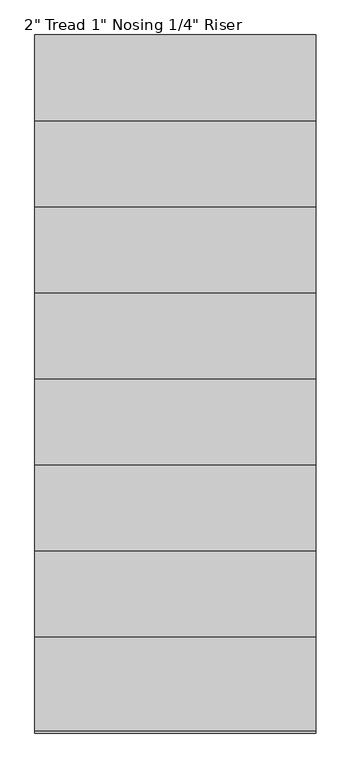
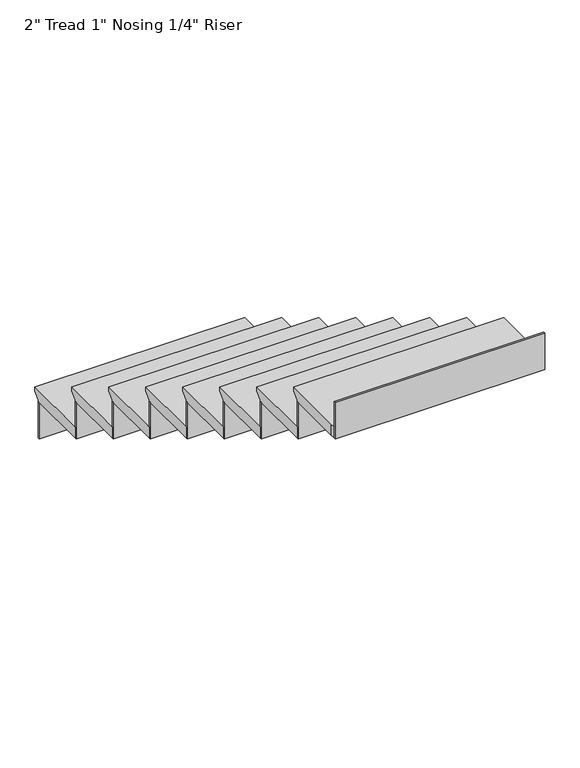
"""IFC4 building model written with IfcOpenShell, lengths in millimetres: stair flight geometry."""

from ifc_helpers import new_model, si_unit, origin, place, context, project, spatial, faceted_brep, source, transform, mapped, element, save


def stair_flight_910e79a6(model_context):
    return source(origin(), model_context, "Body", "Brep", [
        faceted_brep([(16081.5123343, 17121.2483822, 1674.2833333), (16081.5123343, 17121.2483822, 1693.3333333), (16995.9123343, 17121.2483822, 1693.3333333), (16995.9123343, 17121.2483822, 1674.2833333), (16081.5123343, 17095.8483822, 1648.8833333), (16995.9123343, 17095.8483822, 1648.8833333), (16081.5123343, 16816.4483822, 1693.3333333), (16995.9123343, 16816.4483822, 1693.3333333), (16995.9123343, 17095.8483822, 1642.5333333), (16995.9123343, 16816.4483822, 1642.5333333), (16081.5123343, 16816.4483822, 1642.5333333), (16081.5123343, 17095.8483822, 1642.5333333)], [[[0, 1, 2, 3]], [[4, 0, 3, 5]], [[2, 1, 6, 7]], [[8, 9, 10, 11]], [[2, 7, 9, 8, 5, 3]], [[8, 11, 4, 5]], [[6, 1, 0, 4, 11, 10]], [[7, 6, 10, 9]]]),
        faceted_brep([(16081.5123343, 17095.8483822, 1642.5333333), (16081.5123343, 17095.8483822, 1473.2), (16081.5123343, 17089.4983822, 1473.2), (16081.5123343, 17089.4983822, 1642.5333333), (16995.9123343, 17095.8483822, 1642.5333333), (16995.9123343, 17089.4983822, 1642.5333333), (16995.9123343, 17089.4983822, 1473.2), (16995.9123343, 17095.8483822, 1473.2)], [[[0, 1, 2, 3]], [[4, 5, 6, 7]], [[1, 0, 4, 7]], [[2, 1, 7, 6]], [[3, 2, 6, 5]], [[0, 3, 5, 4]]]),
        faceted_brep([(16081.5123343, 16816.4483822, 1811.8666667), (16081.5123343, 16816.4483822, 1642.5333333), (16081.5123343, 16810.0983822, 1642.5333333), (16081.5123343, 16810.0983822, 1811.8666667), (16995.9123343, 16816.4483822, 1811.8666667), (16995.9123343, 16810.0983822, 1811.8666667), (16995.9123343, 16810.0983822, 1642.5333333), (16995.9123343, 16816.4483822, 1642.5333333)], [[[0, 1, 2, 3]], [[4, 5, 6, 7]], [[1, 0, 4, 7]], [[2, 1, 7, 6]], [[3, 2, 6, 5]], [[0, 3, 5, 4]]]),
        faceted_brep([(16995.9123343, 16841.8483822, 1862.6666667), (16081.5123343, 16841.8483822, 1862.6666667), (16081.5123343, 16537.0483822, 1862.6666667), (16995.9123343, 16537.0483822, 1862.6666667), (16995.9123343, 16816.4483822, 1811.8666667), (16995.9123343, 16537.0483822, 1811.8666667), (16081.5123343, 16537.0483822, 1811.8666667), (16081.5123343, 16816.4483822, 1811.8666667), (16995.9123343, 16816.4483822, 1818.2166667), (16995.9123343, 16841.8483822, 1843.6166667), (16081.5123343, 16816.4483822, 1818.2166667), (16081.5123343, 16841.8483822, 1843.6166667)], [[[0, 1, 2, 3]], [[4, 5, 6, 7]], [[0, 3, 5, 4, 8, 9]], [[4, 7, 10, 8]], [[2, 1, 11, 10, 7, 6]], [[3, 2, 6, 5]], [[11, 1, 0, 9]], [[10, 11, 9, 8]]]),
        faceted_brep([(16081.5123343, 16537.0483822, 1981.2), (16081.5123343, 16537.0483822, 1811.8666667), (16081.5123343, 16530.6983822, 1811.8666667), (16081.5123343, 16530.6983822, 1981.2), (16995.9123343, 16537.0483822, 1981.2), (16995.9123343, 16530.6983822, 1981.2), (16995.9123343, 16530.6983822, 1811.8666667), (16995.9123343, 16537.0483822, 1811.8666667)], [[[0, 1, 2, 3]], [[4, 5, 6, 7]], [[1, 0, 4, 7]], [[2, 1, 7, 6]], [[3, 2, 6, 5]], [[0, 3, 5, 4]]]),
        faceted_brep([(16995.9123343, 16562.4483822, 2032.0), (16081.5123343, 16562.4483822, 2032.0), (16081.5123343, 16257.6483822, 2032.0), (16995.9123343, 16257.6483822, 2032.0), (16995.9123343, 16537.0483822, 1981.2), (16995.9123343, 16257.6483822, 1981.2), (16081.5123343, 16257.6483822, 1981.2), (16081.5123343, 16537.0483822, 1981.2), (16995.9123343, 16537.0483822, 1987.55), (16995.9123343, 16562.4483822, 2012.95), (16081.5123343, 16537.0483822, 1987.55), (16081.5123343, 16562.4483822, 2012.95)], [[[0, 1, 2, 3]], [[4, 5, 6, 7]], [[0, 3, 5, 4, 8, 9]], [[4, 7, 10, 8]], [[2, 1, 11, 10, 7, 6]], [[3, 2, 6, 5]], [[11, 1, 0, 9]], [[10, 11, 9, 8]]]),
        faceted_brep([(16081.5123343, 16257.6483822, 2150.5333333), (16081.5123343, 16257.6483822, 1981.2), (16081.5123343, 16251.2983822, 1981.2), (16081.5123343, 16251.2983822, 2150.5333333), (16995.9123343, 16257.6483822, 2150.5333333), (16995.9123343, 16251.2983822, 2150.5333333), (16995.9123343, 16251.2983822, 1981.2), (16995.9123343, 16257.6483822, 1981.2)], [[[0, 1, 2, 3]], [[4, 5, 6, 7]], [[1, 0, 4, 7]], [[2, 1, 7, 6]], [[3, 2, 6, 5]], [[0, 3, 5, 4]]]),
        faceted_brep([(16995.9123343, 16283.0483822, 2201.3333333), (16081.5123343, 16283.0483822, 2201.3333333), (16081.5123343, 15978.2483822, 2201.3333333), (16995.9123343, 15978.2483822, 2201.3333333), (16995.9123343, 16257.6483822, 2150.5333333), (16995.9123343, 15978.2483822, 2150.5333333), (16081.5123343, 15978.2483822, 2150.5333333), (16081.5123343, 16257.6483822, 2150.5333333), (16995.9123343, 16257.6483822, 2156.8833333), (16995.9123343, 16283.0483822, 2182.2833333), (16081.5123343, 16257.6483822, 2156.8833333), (16081.5123343, 16283.0483822, 2182.2833333)], [[[0, 1, 2, 3]], [[4, 5, 6, 7]], [[0, 3, 5, 4, 8, 9]], [[4, 7, 10, 8]], [[2, 1, 11, 10, 7, 6]], [[3, 2, 6, 5]], [[11, 1, 0, 9]], [[10, 11, 9, 8]]]),
        faceted_brep([(16081.5123343, 15978.2483822, 2319.8666667), (16081.5123343, 15978.2483822, 2150.5333333), (16081.5123343, 15971.8983822, 2150.5333333), (16081.5123343, 15971.8983822, 2319.8666667), (16995.9123343, 15978.2483822, 2319.8666667), (16995.9123343, 15971.8983822, 2319.8666667), (16995.9123343, 15971.8983822, 2150.5333333), (16995.9123343, 15978.2483822, 2150.5333333)], [[[0, 1, 2, 3]], [[4, 5, 6, 7]], [[1, 0, 4, 7]], [[2, 1, 7, 6]], [[3, 2, 6, 5]], [[0, 3, 5, 4]]]),
        faceted_brep([(16995.9123343, 16003.6483822, 2370.6666667), (16081.5123343, 16003.6483822, 2370.6666667), (16081.5123343, 15698.8483822, 2370.6666667), (16995.9123343, 15698.8483822, 2370.6666667), (16995.9123343, 15978.2483822, 2319.8666667), (16995.9123343, 15698.8483822, 2319.8666667), (16081.5123343, 15698.8483822, 2319.8666667), (16081.5123343, 15978.2483822, 2319.8666667), (16995.9123343, 15978.2483822, 2326.2166667), (16995.9123343, 16003.6483822, 2351.6166667), (16081.5123343, 15978.2483822, 2326.2166667), (16081.5123343, 16003.6483822, 2351.6166667)], [[[0, 1, 2, 3]], [[4, 5, 6, 7]], [[0, 3, 5, 4, 8, 9]], [[4, 7, 10, 8]], [[2, 1, 11, 10, 7, 6]], [[3, 2, 6, 5]], [[11, 1, 0, 9]], [[10, 11, 9, 8]]]),
        faceted_brep([(16081.5123343, 15698.8483822, 2489.2), (16081.5123343, 15698.8483822, 2319.8666667), (16081.5123343, 15692.4983822, 2319.8666667), (16081.5123343, 15692.4983822, 2489.2), (16995.9123343, 15698.8483822, 2489.2), (16995.9123343, 15692.4983822, 2489.2), (16995.9123343, 15692.4983822, 2319.8666667), (16995.9123343, 15698.8483822, 2319.8666667)], [[[0, 1, 2, 3]], [[4, 5, 6, 7]], [[1, 0, 4, 7]], [[2, 1, 7, 6]], [[3, 2, 6, 5]], [[0, 3, 5, 4]]]),
        faceted_brep([(16995.9123343, 15724.2483822, 2540.0), (16081.5123343, 15724.2483822, 2540.0), (16081.5123343, 15419.4483822, 2540.0), (16995.9123343, 15419.4483822, 2540.0), (16995.9123343, 15698.8483822, 2489.2), (16995.9123343, 15419.4483822, 2489.2), (16081.5123343, 15419.4483822, 2489.2), (16081.5123343, 15698.8483822, 2489.2), (16995.9123343, 15698.8483822, 2495.55), (16995.9123343, 15724.2483822, 2520.95), (16081.5123343, 15698.8483822, 2495.55), (16081.5123343, 15724.2483822, 2520.95)], [[[0, 1, 2, 3]], [[4, 5, 6, 7]], [[0, 3, 5, 4, 8, 9]], [[4, 7, 10, 8]], [[2, 1, 11, 10, 7, 6]], [[3, 2, 6, 5]], [[11, 1, 0, 9]], [[10, 11, 9, 8]]]),
        faceted_brep([(16081.5123343, 15419.4483822, 2658.5333333), (16081.5123343, 15419.4483822, 2489.2), (16081.5123343, 15413.0983822, 2489.2), (16081.5123343, 15413.0983822, 2658.5333333), (16995.9123343, 15419.4483822, 2658.5333333), (16995.9123343, 15413.0983822, 2658.5333333), (16995.9123343, 15413.0983822, 2489.2), (16995.9123343, 15419.4483822, 2489.2)], [[[0, 1, 2, 3]], [[4, 5, 6, 7]], [[1, 0, 4, 7]], [[2, 1, 7, 6]], [[3, 2, 6, 5]], [[0, 3, 5, 4]]]),
        faceted_brep([(16995.9123343, 15444.8483822, 2709.3333333), (16081.5123343, 15444.8483822, 2709.3333333), (16081.5123343, 15140.0483822, 2709.3333333), (16995.9123343, 15140.0483822, 2709.3333333), (16995.9123343, 15419.4483822, 2658.5333333), (16995.9123343, 15140.0483822, 2658.5333333), (16081.5123343, 15140.0483822, 2658.5333333), (16081.5123343, 15419.4483822, 2658.5333333), (16995.9123343, 15419.4483822, 2664.8833333), (16995.9123343, 15444.8483822, 2690.2833333), (16081.5123343, 15419.4483822, 2664.8833333), (16081.5123343, 15444.8483822, 2690.2833333)], [[[0, 1, 2, 3]], [[4, 5, 6, 7]], [[0, 3, 5, 4, 8, 9]], [[4, 7, 10, 8]], [[2, 1, 11, 10, 7, 6]], [[3, 2, 6, 5]], [[11, 1, 0, 9]], [[10, 11, 9, 8]]]),
        faceted_brep([(16081.5123343, 14860.6483822, 2997.2), (16081.5123343, 14860.6483822, 2827.8666667), (16081.5123343, 14854.2983822, 2827.8666667), (16081.5123343, 14854.2983822, 2997.2), (16995.9123343, 14860.6483822, 2997.2), (16995.9123343, 14854.2983822, 2997.2), (16995.9123343, 14854.2983822, 2827.8666667), (16995.9123343, 14860.6483822, 2827.8666667)], [[[0, 1, 2, 3]], [[4, 5, 6, 7]], [[1, 0, 4, 7]], [[2, 1, 7, 6]], [[3, 2, 6, 5]], [[0, 3, 5, 4]]]),
        faceted_brep([(16081.5123343, 15140.0483822, 2827.8666667), (16081.5123343, 15140.0483822, 2658.5333333), (16081.5123343, 15133.6983822, 2658.5333333), (16081.5123343, 15133.6983822, 2827.8666667), (16995.9123343, 15140.0483822, 2827.8666667), (16995.9123343, 15133.6983822, 2827.8666667), (16995.9123343, 15133.6983822, 2658.5333333), (16995.9123343, 15140.0483822, 2658.5333333)], [[[0, 1, 2, 3]], [[4, 5, 6, 7]], [[1, 0, 4, 7]], [[2, 1, 7, 6]], [[3, 2, 6, 5]], [[0, 3, 5, 4]]]),
        faceted_brep([(16995.9123343, 14860.6483822, 2878.6666667), (16995.9123343, 14886.0483822, 2878.6666667), (16995.9123343, 15165.4483822, 2878.6666667), (16081.5123343, 15165.4483822, 2878.6666667), (16081.5123343, 14886.0483822, 2878.6666667), (16081.5123343, 14860.6483822, 2878.6666667), (16995.9123343, 14886.0483822, 2827.8666667), (16995.9123343, 14860.6483822, 2827.8666667), (16081.5123343, 14860.6483822, 2827.8666667), (16081.5123343, 14886.0483822, 2827.8666667), (16081.5123343, 15140.0483822, 2827.8666667), (16995.9123343, 15140.0483822, 2827.8666667), (16995.9123343, 15140.0483822, 2834.2166667), (16995.9123343, 15165.4483822, 2859.6166667), (16081.5123343, 15140.0483822, 2834.2166667), (16081.5123343, 15165.4483822, 2859.6166667)], [[[0, 1, 2, 3, 4, 5]], [[6, 7, 8, 9, 10, 11]], [[1, 0, 7, 6]], [[2, 1, 6, 11, 12, 13]], [[11, 10, 14, 12]], [[4, 3, 15, 14, 10, 9]], [[5, 4, 9, 8]], [[0, 5, 8, 7]], [[15, 3, 2, 13]], [[14, 15, 13, 12]]]),
    ])


if __name__ == "__main__":
    model = new_model("IFC4")
    model_context = context("Model", 3, world=origin())
    ifc_project = project(units=[si_unit("LENGTHUNIT", "METRE", prefix="MILLI")], contexts=[model_context])
    site = spatial("IfcSite", under=ifc_project)
    building = spatial("IfcBuilding", under=site)
    placement = place(None, origin())
    stair_flight_shape = stair_flight_910e79a6(model_context)
    element("IfcStairFlight", 1, ObjectType="2\" Tread 1\" Nosing 1/4\" Riser", at=placement, inside=building, context=model_context, shape_type="MappedRepresentation", body=[
        mapped(stair_flight_shape, transform((0.0, 0.0, 0.0), x_axis=(1.0, 0.0, 0.0), y_axis=(0.0, 1.0, 0.0), z_axis=(0.0, 0.0, 1.0))),
    ])
    save(model, "model.ifc")
